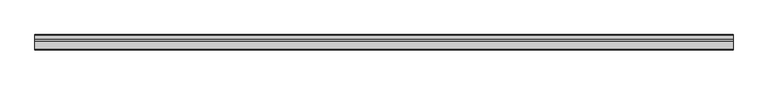
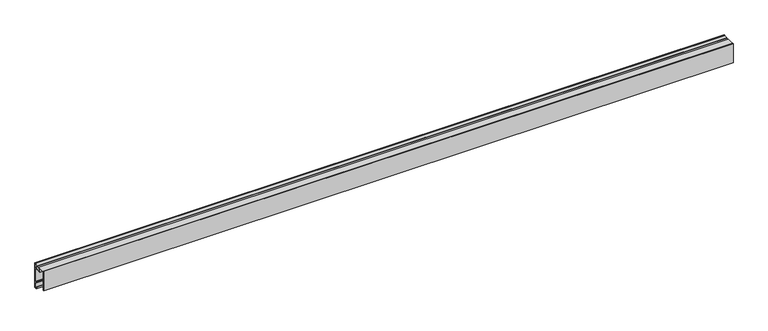
"""IFC4 building model written with IfcOpenShell, lengths in millimetres: proxy geometry, Generic Models 6:Generic Models 2:318829:Generic Models 2:318829 : Generic Models 6:Generic Models 2:318829:1 : Generic Models 6:Generic Models 2:318829:Generic Models 2:318829 : Generic Models 6:Generic Models 2:318829:300683."""

from ifc_helpers import new_model, si_unit, frame, origin, place, context, project, spatial, polyline, outline, extrude, source, transform, mapped, element, save


def generic_models_90b0fa55(model_context):
    return source(origin(), model_context, "Body", "SweptSolid", [
        extrude(outline(polyline([(-579037.334754, 3698.478125), (-579020.7824978, 3698.478125), (-579020.7824978, 3693.7806264), (-579022.7079133, 3693.7806264), (-579022.7079133, 3691.3993764), (-579020.7824978, 3691.3993764), (-579020.7824978, 3686.7018777), (-579037.334754, 3686.7018777), (-579037.334754, 3691.3993764), (-579035.4093386, 3691.3993764), (-579035.4093386, 3693.7806264), (-579037.334754, 3693.7806264), (-579037.334754, 3698.478125)])), frame((590317.0242239, 0.0, 0.0), z_axis=(1.0, 0.0, 0.0), x_axis=(0.0, 1.0, 0.0)), (0.0, 0.0, 1.0), 2438.4),
        extrude(outline(polyline([(-579010.8549878, 3700.4625), (-579010.8549878, 3702.05), (-579009.2674878, 3702.05), (-579009.2674878, 3610.05), (-579017.7138594, 3610.05), (-579017.7138594, 3614.4373266), (-579016.1263594, 3614.4373266), (-579016.1263594, 3611.6375), (-579010.8549878, 3611.6375), (-579010.8549878, 3631.6375), (-579017.7138594, 3631.6375), (-579017.7138594, 3636.0248266), (-579016.1263594, 3636.0248266), (-579016.1263594, 3633.225), (-579010.8549878, 3633.225), (-579010.8549878, 3684.7175027), (-579024.5528103, 3684.7175027), (-579024.5528103, 3686.3050027), (-579020.3856228, 3686.3050027), (-579020.3856228, 3691.7962514), (-579022.3110383, 3691.7962514), (-579022.3110383, 3693.3837514), (-579020.3856228, 3693.3837514), (-579020.3856228, 3698.875), (-579024.5528103, 3698.875), (-579024.5528103, 3700.4625), (-579010.8549878, 3700.4625)]), holes=[polyline([(-579010.8549878, 3686.3050027), (-579010.8549878, 3698.875), (-579018.7981228, 3698.875), (-579018.7981228, 3686.3050027), (-579010.8549878, 3686.3050027)])]), frame((590317.0242239, 0.0, 0.0), z_axis=(1.0, 0.0, 0.0), x_axis=(0.0, 1.0, 0.0)), (0.0, 0.0, 1.0), 2438.4),
        extrude(outline(polyline([(-579060.5523979, 3631.6375), (-579060.5523979, 3630.05), (-579063.2674878, 3630.05), (-579063.2674878, 3702.05), (-579061.6799878, 3702.05), (-579061.6799878, 3700.4625), (-579033.5644415, 3700.4625), (-579033.5644415, 3698.875), (-579037.731629, 3698.875), (-579037.731629, 3693.3837514), (-579035.8062136, 3693.3837514), (-579035.8062136, 3691.7962514), (-579037.731629, 3691.7962514), (-579037.731629, 3686.3050027), (-579033.5644415, 3686.3050027), (-579033.5644415, 3684.7175027), (-579039.319129, 3684.7175027), (-579039.319129, 3698.875), (-579061.6799878, 3698.875), (-579061.6799878, 3631.6375), (-579060.5523979, 3631.6375)])), frame((590317.0242239, 0.0, 0.0), z_axis=(1.0, 0.0, 0.0), x_axis=(0.0, 1.0, 0.0)), (0.0, 0.0, 1.0), 2438.4),
    ])


if __name__ == "__main__":
    model = new_model("IFC4")
    model_context = context("Model", 3, world=origin())
    ifc_project = project(units=[si_unit("LENGTHUNIT", "METRE", prefix="MILLI")], contexts=[model_context])
    site = spatial("IfcSite", under=ifc_project)
    building = spatial("IfcBuilding", under=site)
    placement = place(None, origin())
    generic_models_shape = generic_models_90b0fa55(model_context)
    element("IfcBuildingElementProxy", 1, Name="Generic Models 6:Generic Models 2:318829:Generic Models 2:318829 : Generic Models 6:Generic Models 2:318829:1 : Generic Models 6:Generic Models 2:318829:Generic Models 2:318829 : Generic Models 6:Generic Models 2:318829:300683", ObjectType="Generic Models 6:Generic Models 2:318829:Generic Models 2:318829 : Generic Models 6:Generic Models 2:318829:1 : Generic Models 6:Generic Models 2:318829:Generic Models 2:318829 : Generic Models 6:Generic Models 2:318829:300683", at=placement, inside=building, context=model_context, shape_type="MappedRepresentation", body=[
        mapped(generic_models_shape, transform((0.0, 0.0, 0.0), x_axis=(1.0, 0.0, 0.0), y_axis=(0.0, 1.0, 0.0), z_axis=(0.0, 0.0, 1.0))),
    ])
    save(model, "model.ifc")

# Revit data of these elements
# Type "Generic Models 6:Generic Models 2:318829:Generic Models 2:318829 : Generic Models 6:Generic Models 2:318829:1 : Generic Models 6:Generic Models 2:318829:Generic Models 2:318829 : Generic Models 6:Generic Models 2:318829:300683"
#   NameOverride = "Generic Models 6:Generic Models 2:318829:Generic Models 2:318829 : Generic Models 6:Generic Models 2:318829:300683"
#   ObjectTypeOverride = "Generic Models 2:318829 : Generic Models 6:Generic Models 2:318829"
#   Reference = "Generic Models 2"
#   Tag = "300683"
# Element 1 (IfcBuildingElementProxy, "Generic Models 6:Generic Models 2:318829:Generic Models 2:318829 : Generic Models 6:Generic Models 2:318829:1 : Generic Models 6:Generic Models 2:318829:Generic Models 2:318829 : Generic Models 6:Generic Models 2:318829:300683")
#   Materials on its faces: "THERMAL BROKEN ALUMINUM STOREFRONT FOR POLYCARBONATE"
# Materials
#   "THERMAL BROKEN ALUMINUM STOREFRONT FOR POLYCARBONATE": class "Unassigned", colour RGB 244 244 244, transparency 0, Keynote = "M07611300.01", Cost = 0
